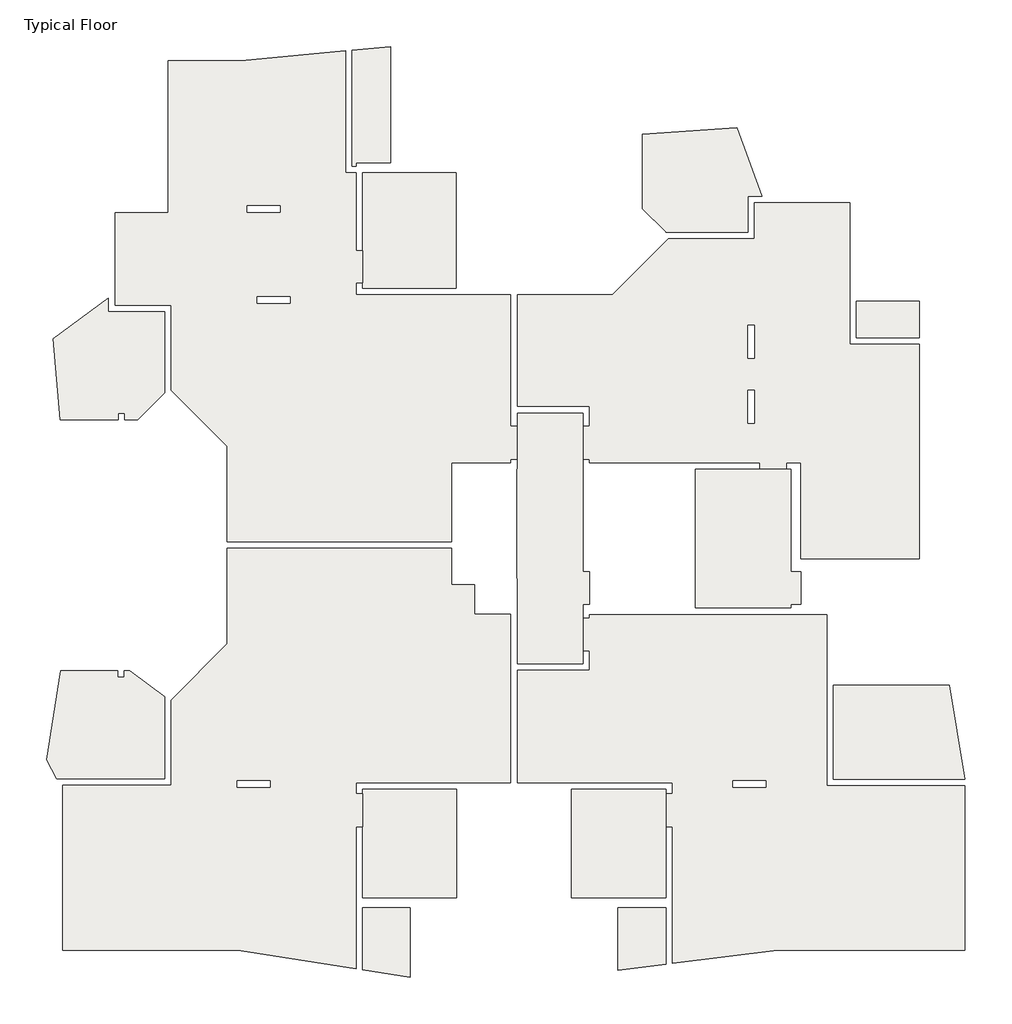
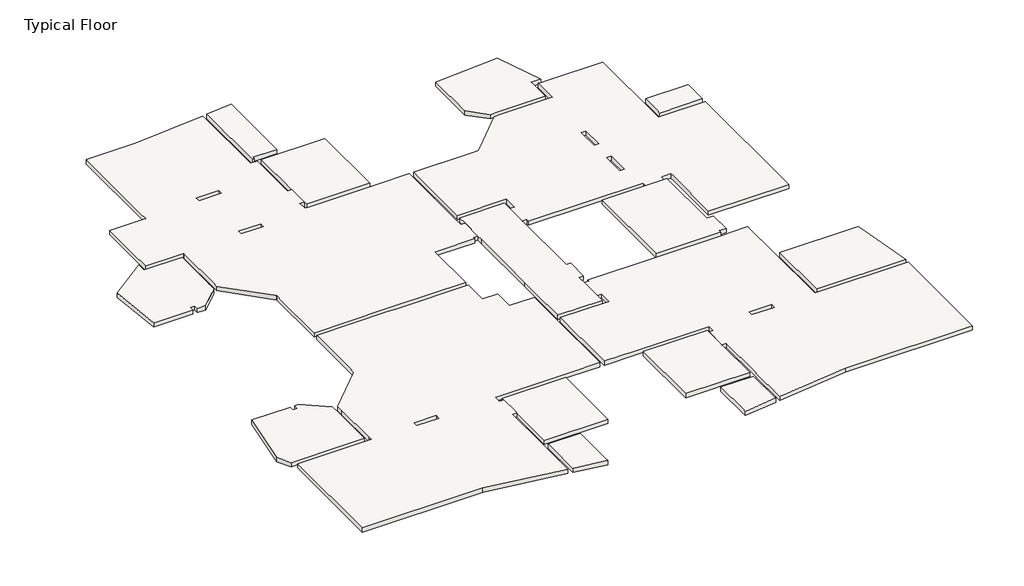
# One storey: 17 slabs.
"""IFC4 building model written with IfcOpenShell, lengths in millimetres."""

from ifc_helpers import new_model, si_unit, origin, place, context, project, spatial, faceted_brep, element, save

model = new_model("IFC4")

# Units and contexts
model_context = context("Model", 3, world=origin())
ifc_project = project(units=[si_unit("LENGTHUNIT", "METRE", prefix="MILLI")], contexts=[model_context])

# Site, building, storey
site = spatial("IfcSite", under=ifc_project)
building = spatial("IfcBuilding", under=site)
storey = spatial("IfcBuildingStorey", under=building, Name="Typical Floor", Elevation=2850.0)

# Slabs
placement = place(None, origin())
element("IfcSlab", 1, ObjectType="20", at=placement, inside=storey, context=model_context, shape_type="Brep", body=[
    faceted_brep([(-15286.5645409, -11765.3513235, 2650.0), (-18561.5127169, -11765.3513235, 2650.0), (-18869.0821124, -11186.8974215, 2650.0), (-18443.4032212, -8499.2666773, 2650.0), (-16708.8112897, -8499.2666773, 2650.0), (-16708.8112897, -8694.3603589, 2650.0), (-16508.8112897, -8694.3603589, 2650.0), (-16508.8112897, -8499.2666773, 2650.0), (-16353.4071605, -8499.2666773, 2650.0), (-15286.5645409, -9274.373211, 2650.0), (-18561.5127169, -11765.3513235, 2850.0), (-18379.347479, -11765.3513235, 2850.0), (-15486.5645409, -11765.3513235, 2850.0), (-15286.5645409, -11765.3513235, 2850.0), (-15286.5645409, -9691.9014804, 2850.0), (-15286.5645409, -9291.9014804, 2850.0), (-15286.5645409, -9274.373211, 2850.0), (-16353.4071605, -8499.2666773, 2850.0), (-16508.8112897, -8499.2666773, 2850.0), (-16508.8112897, -8694.3603589, 2850.0), (-16708.8112897, -8694.3603589, 2850.0), (-16708.8112897, -8499.2666773, 2850.0), (-18443.4032212, -8499.2666773, 2850.0), (-18869.0821124, -11186.8974215, 2850.0)], [[[0, 1, 2, 3, 4, 5, 6, 7, 8, 9]], [[10, 11, 12, 13, 14, 15, 16, 17, 18, 19, 20, 21, 22, 23]], [[1, 0, 13, 12, 11, 10]], [[2, 1, 10, 23]], [[3, 2, 23, 22]], [[4, 3, 22, 21]], [[5, 4, 21, 20]], [[6, 5, 20, 19]], [[7, 6, 19, 18]], [[8, 7, 18, 17]], [[9, 8, 17, 16]], [[0, 9, 16, 15, 14, 13]]]),
])
element("IfcSlab", 2, ObjectType="20", at=placement, inside=storey, context=model_context, shape_type="Brep", body=[
    faceted_brep([(-6440.6856227, -12083.2914692, 2650.0), (-6440.6856227, -15367.9244771, 2650.0), (-9283.9897454, -15367.9244771, 2650.0), (-9283.9897454, -13219.4691321, 2650.0), (-9283.9897454, -12214.5716558, 2650.0), (-9283.9897454, -12083.2914692, 2650.0), (-6440.6856227, -12083.2914692, 2850.0), (-9283.9897454, -12083.2914692, 2850.0), (-9283.9897454, -12214.5716558, 2850.0), (-9283.9897454, -13219.4691321, 2850.0), (-9283.9897454, -15367.9244771, 2850.0), (-6440.6856227, -15367.9244771, 2850.0)], [[[0, 1, 2, 3, 4, 5]], [[6, 7, 8, 9, 10, 11]], [[1, 0, 6, 11]], [[2, 1, 11, 10]], [[5, 4, 3, 2, 10, 9, 8, 7]], [[0, 5, 7, 6]]]),
])
element("IfcSlab", 3, ObjectType="20", at=placement, inside=storey, context=model_context, shape_type="Brep", body=[
    faceted_brep([(-87.6035477, -12083.2914692, 2650.0), (-87.6035477, -12214.5716558, 2650.0), (-87.6035477, -13219.4691321, 2650.0), (-87.6035477, -15367.9244771, 2650.0), (-2954.5902544, -15367.9244771, 2650.0), (-2954.5902544, -12083.2914692, 2650.0), (-87.6035477, -12083.2914692, 2850.0), (-2954.5902544, -12083.2914692, 2850.0), (-2954.5902544, -15367.9244771, 2850.0), (-87.6035477, -15367.9244771, 2850.0), (-87.6035477, -13219.4691321, 2850.0), (-87.6035477, -12214.5716558, 2850.0)], [[[0, 1, 2, 3, 4, 5]], [[6, 7, 8, 9, 10, 11]], [[3, 2, 1, 0, 6, 11, 10, 9]], [[4, 3, 9, 8]], [[5, 4, 8, 7]], [[0, 5, 7, 6]]]),
])
element("IfcSlab", 4, ObjectType="20", at=placement, inside=storey, context=model_context, shape_type="Brep", body=[
    faceted_brep([(-9283.9897454, -15667.9244771, 2650.0), (-7844.4831614, -15667.9244771, 2650.0), (-7844.4831614, -17786.8222268, 2650.0), (-9283.9897454, -17557.8098157, 2650.0), (-9283.9897454, -15667.9244771, 2850.0), (-9283.9897454, -17344.4159012, 2850.0), (-9283.9897454, -17557.8098157, 2850.0), (-7844.4831614, -17786.8222268, 2850.0), (-7844.4831614, -17605.2464942, 2850.0), (-7844.4831614, -15667.9244771, 2850.0)], [[[0, 1, 2, 3]], [[4, 5, 6, 7, 8, 9]], [[1, 0, 4, 9]], [[2, 1, 9, 8, 7]], [[3, 2, 7, 6]], [[0, 3, 6, 5, 4]]]),
])
element("IfcSlab", 5, ObjectType="20", at=placement, inside=storey, context=model_context, shape_type="Brep", body=[
    faceted_brep([(-18379.347479, -16969.7313812, 2650.0), (-18379.347479, -11965.3513235, 2650.0), (-15086.5645409, -11965.3513235, 2650.0), (-15086.5645409, -11765.3513235, 2650.0), (-15089.2187138, -11765.3513235, 2650.0), (-15089.2187138, -9691.9014804, 2650.0), (-15086.5645409, -9691.9014804, 2650.0), (-15086.5645409, -9380.9473819, 2650.0), (-13387.4363964, -7681.8192373, 2650.0), (-13387.4363964, -7281.8192373, 2650.0), (-13387.4363964, -4887.4320305, 2650.0), (-13387.4363964, -4787.4320305, 2650.0), (-6597.6379386, -4787.4320305, 2650.0), (-6597.6379386, -5683.2914692, 2650.0), (-6597.6379386, -5883.2914692, 2650.0), (-5897.6379386, -5883.2914692, 2650.0), (-5897.6379386, -6583.2914692, 2650.0), (-5897.6379386, -6783.2914692, 2650.0), (-4797.6379386, -6783.2914692, 2650.0), (-4797.6379386, -11883.2914692, 2650.0), (-6190.6856227, -11883.2914692, 2650.0), (-9283.9897454, -11883.2914692, 2650.0), (-9483.9897454, -11883.2914692, 2650.0), (-9483.9897454, -12214.5716558, 2650.0), (-9283.9897454, -12214.5716558, 2650.0), (-9283.9897454, -13079.4691321, 2650.0), (-9283.9897454, -13219.4691321, 2650.0), (-9483.9897454, -13219.4691321, 2650.0), (-9483.9897454, -15367.9244771, 2650.0), (-9483.9897454, -15667.9244771, 2650.0), (-9483.9897454, -17344.4159012, 2650.0), (-9483.9897454, -17526.0844321, 2650.0), (-12973.5990213, -16973.3846199, 2650.0), (-12973.5990213, -16969.7313812, 2650.0), (-13373.5990213, -16969.7313812, 2650.0), (-12084.0109343, -12024.8863444, 2650.0), (-12084.0109343, -11824.8863444, 2650.0), (-13084.0109343, -11824.8863444, 2650.0), (-13084.0109343, -12024.8863444, 2650.0), (-18379.347479, -11965.3513235, 2850.0), (-18379.347479, -12165.3513235, 2850.0), (-18379.347479, -16769.7313812, 2850.0), (-18379.347479, -16969.7313812, 2850.0), (-13373.5990213, -16969.7313812, 2850.0), (-12973.5990213, -16969.7313812, 2850.0), (-12973.5990213, -16973.3846199, 2850.0), (-9483.9897454, -17526.0844321, 2850.0), (-9483.9897454, -17344.4159012, 2850.0), (-9483.9897454, -15667.9244771, 2850.0), (-9483.9897454, -15367.9244771, 2850.0), (-9483.9897454, -13219.4691321, 2850.0), (-9283.9897454, -13219.4691321, 2850.0), (-9283.9897454, -13079.4691321, 2850.0), (-9283.9897454, -12214.5716558, 2850.0), (-9483.9897454, -12214.5716558, 2850.0), (-9483.9897454, -11883.2914692, 2850.0), (-9283.9897454, -11883.2914692, 2850.0), (-6190.6856227, -11883.2914692, 2850.0), (-4797.6379386, -11883.2914692, 2850.0), (-4797.6379386, -11683.2914692, 2850.0), (-4797.6379386, -8483.2914692, 2850.0), (-4797.6379386, -8283.2914692, 2850.0), (-4797.6379386, -6783.2914692, 2850.0), (-5897.6379386, -6783.2914692, 2850.0), (-5897.6379386, -6583.2914692, 2850.0), (-5897.6379386, -5883.2914692, 2850.0), (-6597.6379386, -5883.2914692, 2850.0), (-6597.6379386, -5683.2914692, 2850.0), (-6597.6379386, -4787.4320305, 2850.0), (-9795.9008278, -4787.4320305, 2850.0), (-10195.9008278, -4787.4320305, 2850.0), (-13387.4363964, -4787.4320305, 2850.0), (-13387.4363964, -4887.4320305, 2850.0), (-13387.4363964, -7281.8192373, 2850.0), (-13387.4363964, -7681.8192373, 2850.0), (-15086.5645409, -9380.9473819, 2850.0), (-15086.5645409, -9691.9014804, 2850.0), (-15089.2187138, -9691.9014804, 2850.0), (-15089.2187138, -11765.3513235, 2850.0), (-15086.5645409, -11765.3513235, 2850.0), (-15086.5645409, -11965.3513235, 2850.0), (-15486.5645409, -11965.3513235, 2850.0), (-12084.0109343, -11824.8863444, 2850.0), (-12084.0109343, -12024.8863444, 2850.0), (-13084.0109343, -12024.8863444, 2850.0), (-13084.0109343, -11824.8863444, 2850.0)], [[[0, 1, 2, 3, 4, 5, 6, 7, 8, 9, 10, 11, 12, 13, 14, 15, 16, 17, 18, 19, 20, 21, 22, 23, 24, 25, 26, 27, 28, 29, 30, 31, 32, 33, 34], [35, 36, 37, 38]], [[39, 40, 41, 42, 43, 44, 45, 46, 47, 48, 49, 50, 51, 52, 53, 54, 55, 56, 57, 58, 59, 60, 61, 62, 63, 64, 65, 66, 67, 68, 69, 70, 71, 72, 73, 74, 75, 76, 77, 78, 79, 80, 81], [82, 83, 84, 85]], [[1, 0, 42, 41, 40, 39]], [[1, 39, 81, 80, 2]], [[77, 5, 4, 78]], [[74, 8, 7, 75]], [[8, 74, 73, 72, 71, 11, 10, 9]], [[12, 11, 71, 70, 69, 68]], [[12, 68, 67, 66, 14, 13]], [[15, 14, 66, 65]], [[15, 65, 64, 63, 17, 16]], [[18, 17, 63, 62]], [[19, 18, 62, 61, 60, 59, 58]], [[19, 58, 57, 56, 55, 22, 21, 20]], [[23, 22, 55, 54]], [[24, 23, 54, 53]], [[25, 24, 53, 52]], [[26, 25, 52, 51]], [[27, 26, 51, 50]], [[27, 50, 49, 48, 47, 46, 31, 30, 29, 28]], [[32, 31, 46, 45]], [[33, 32, 45, 44]], [[33, 44, 43, 42, 0, 34]], [[6, 76, 75, 7]], [[76, 6, 5, 77]], [[3, 79, 78, 4]], [[79, 3, 2, 80]], [[35, 83, 82, 36]], [[83, 35, 38, 84]], [[84, 38, 37, 85]], [[85, 37, 36, 82]]]),
])
element("IfcSlab", 6, ObjectType="20", at=placement, inside=storey, context=model_context, shape_type="Brep", body=[
    faceted_brep([(8500.876934, -8926.3350173, 2650.0), (8977.0164469, -11773.6548619, 2650.0), (8977.0164469, -11783.2914692, 2650.0), (4985.5431075, -11783.2914692, 2650.0), (4985.5431075, -8926.3350173, 2650.0), (8500.876934, -8926.3350173, 2850.0), (4985.5431075, -8926.3350173, 2850.0), (4985.5431075, -9026.3350173, 2850.0), (4985.5431075, -11583.2914692, 2850.0), (4985.5431075, -11783.2914692, 2850.0), (8977.0164469, -11783.2914692, 2850.0), (8977.0164469, -11773.6548619, 2850.0)], [[[0, 1, 2, 3, 4]], [[5, 6, 7, 8, 9, 10, 11]], [[1, 0, 5, 11]], [[2, 1, 11, 10]], [[3, 2, 10, 9]], [[4, 3, 9, 8, 7, 6]], [[0, 4, 6, 5]]]),
])
element("IfcSlab", 7, ObjectType="20", at=placement, inside=storey, context=model_context, shape_type="Brep", body=[
    faceted_brep([(-4597.6379386, -8483.2914692, 2650.0), (-2403.3824041, -8483.2914692, 2650.0), (-2403.3824041, -8283.2914692, 2650.0), (-2403.3824041, -7883.2914692, 2650.0), (-2603.3824041, -7883.2914692, 2650.0), (-2603.3824041, -6894.6673257, 2650.0), (-2403.3824041, -6894.6673257, 2650.0), (-2403.3824041, -6790.494584, 2650.0), (4785.5431075, -6790.494584, 2650.0), (4785.5431075, -6990.494584, 2650.0), (4785.5431075, -8626.3350173, 2650.0), (4785.5431075, -9026.3350173, 2650.0), (4785.5431075, -11583.2914692, 2650.0), (4785.5431075, -11983.2914692, 2650.0), (4985.5431075, -11983.2914692, 2650.0), (8977.0164469, -11983.2914692, 2650.0), (8977.0164469, -16969.7313812, 2650.0), (3695.6052151, -16969.7313812, 2650.0), (3295.6052151, -16969.7313812, 2650.0), (3289.488953, -16969.7313812, 2650.0), (112.3964523, -17359.8292888, 2650.0), (112.3964523, -17190.4678354, 2650.0), (112.3964523, -15667.9244771, 2650.0), (112.3964523, -15367.9244771, 2650.0), (112.3964523, -13219.4691321, 2650.0), (-87.6035477, -13219.4691321, 2650.0), (-87.6035477, -12214.5716558, 2650.0), (112.3964523, -12214.5716558, 2650.0), (112.3964523, -11883.2914692, 2650.0), (-87.6035477, -11883.2914692, 2650.0), (-3204.5902544, -11883.2914692, 2650.0), (-4597.6379386, -11883.2914692, 2650.0), (2945.6091526, -11824.8863444, 2650.0), (1945.6091526, -11824.8863444, 2650.0), (1945.6091526, -12024.8863444, 2650.0), (2945.6091526, -12024.8863444, 2650.0), (-2403.3824041, -8483.2914692, 2850.0), (-4597.6379386, -8483.2914692, 2850.0), (-4597.6379386, -11683.2914692, 2850.0), (-4597.6379386, -11883.2914692, 2850.0), (-3204.5902544, -11883.2914692, 2850.0), (-87.6035477, -11883.2914692, 2850.0), (112.3964523, -11883.2914692, 2850.0), (112.3964523, -12214.5716558, 2850.0), (-87.6035477, -12214.5716558, 2850.0), (-87.6035477, -13219.4691321, 2850.0), (112.3964523, -13219.4691321, 2850.0), (112.3964523, -15367.9244771, 2850.0), (112.3964523, -15667.9244771, 2850.0), (112.3964523, -17190.4678354, 2850.0), (112.3964523, -17359.8292888, 2850.0), (3289.488953, -16969.7313812, 2850.0), (3295.6052151, -16969.7313812, 2850.0), (3695.6052151, -16969.7313812, 2850.0), (8977.0164469, -16969.7313812, 2850.0), (8977.0164469, -16771.5953491, 2850.0), (8977.0164469, -12165.3513235, 2850.0), (8977.0164469, -11983.2914692, 2850.0), (4985.5431075, -11983.2914692, 2850.0), (4785.5431075, -11983.2914692, 2850.0), (4785.5431075, -11583.2914692, 2850.0), (4785.5431075, -9026.3350173, 2850.0), (4785.5431075, -8626.3350173, 2850.0), (4785.5431075, -6990.494584, 2850.0), (4785.5431075, -6790.494584, 2850.0), (3996.1514357, -6790.494584, 2850.0), (3696.1514357, -6790.494584, 2850.0), (-2403.3824041, -6790.494584, 2850.0), (-2403.3824041, -6894.6673257, 2850.0), (-2603.3824041, -6894.6673257, 2850.0), (-2603.3824041, -7883.2914692, 2850.0), (-2403.3824041, -7883.2914692, 2850.0), (-2403.3824041, -8283.2914692, 2850.0), (1945.6091526, -11824.8863444, 2850.0), (2945.6091526, -11824.8863444, 2850.0), (2945.6091526, -12024.8863444, 2850.0), (1945.6091526, -12024.8863444, 2850.0)], [[[0, 1, 2, 3, 4, 5, 6, 7, 8, 9, 10, 11, 12, 13, 14, 15, 16, 17, 18, 19, 20, 21, 22, 23, 24, 25, 26, 27, 28, 29, 30, 31], [32, 33, 34, 35]], [[36, 37, 38, 39, 40, 41, 42, 43, 44, 45, 46, 47, 48, 49, 50, 51, 52, 53, 54, 55, 56, 57, 58, 59, 60, 61, 62, 63, 64, 65, 66, 67, 68, 69, 70, 71, 72], [73, 74, 75, 76]], [[1, 0, 37, 36]], [[1, 36, 72, 71, 3, 2]], [[4, 3, 71, 70]], [[5, 4, 70, 69]], [[6, 5, 69, 68]], [[7, 6, 68, 67]], [[8, 7, 67, 66, 65, 64]], [[8, 64, 63, 62, 61, 60, 59, 13, 12, 11, 10, 9]], [[13, 59, 58, 57, 15, 14]], [[16, 15, 57, 56, 55, 54]], [[16, 54, 53, 52, 18, 17]], [[19, 18, 52, 51]], [[20, 19, 51, 50]], [[20, 50, 49, 48, 47, 46, 24, 23, 22, 21]], [[25, 24, 46, 45]], [[26, 25, 45, 44]], [[27, 26, 44, 43]], [[28, 27, 43, 42]], [[28, 42, 41, 40, 39, 31, 30, 29]], [[0, 31, 39, 38, 37]], [[33, 32, 74, 73]], [[34, 33, 73, 76]], [[35, 34, 76, 75]], [[32, 35, 75, 74]]]),
])
element("IfcSlab", 8, ObjectType="20", at=placement, inside=storey, context=model_context, shape_type="Brep", body=[
    faceted_brep([(7591.3944084, 2705.1624293, 2650.0), (7591.3944084, 1595.5159248, 2650.0), (5684.9828456, 1595.5159248, 2650.0), (5684.9828456, 2705.1624293, 2650.0), (7591.3944084, 2705.1624293, 2850.0), (5684.9828456, 2705.1624293, 2850.0), (5684.9828456, 1795.5159248, 2850.0), (5684.9828456, 1595.5159248, 2850.0), (7591.3944084, 1595.5159248, 2850.0)], [[[0, 1, 2, 3]], [[4, 5, 6, 7, 8]], [[1, 0, 4, 8]], [[2, 1, 8, 7]], [[3, 2, 7, 6, 5]], [[0, 3, 5, 4]]]),
])
element("IfcSlab", 9, ObjectType="20", at=placement, inside=storey, context=model_context, shape_type="Brep", body=[
    faceted_brep([(-6450.1625371, 3095.9323955, 2650.0), (-9290.6856227, 3095.9323955, 2650.0), (-9290.6856227, 3262.2142639, 2650.0), (-9290.6856227, 4237.8899275, 2650.0), (-9290.6856227, 6597.8899275, 2650.0), (-6450.1625371, 6597.8899275, 2650.0), (-6450.1625371, 3095.9323955, 2850.0), (-6450.1625371, 6597.8899275, 2850.0), (-9290.6856227, 6597.8899275, 2850.0), (-9290.6856227, 4237.8899275, 2850.0), (-9290.6856227, 3262.2142639, 2850.0), (-9290.6856227, 3095.9323955, 2850.0)], [[[0, 1, 2, 3, 4, 5]], [[6, 7, 8, 9, 10, 11]], [[1, 0, 6, 11]], [[4, 3, 2, 1, 11, 10, 9, 8]], [[5, 4, 8, 7]], [[0, 5, 7, 6]]]),
])
element("IfcSlab", 10, ObjectType="20", at=placement, inside=storey, context=model_context, shape_type="Brep", body=[
    faceted_brep([(-9490.6856227, 4237.8899275, 2650.0), (-9290.6856227, 4237.8899275, 2650.0), (-9290.6856227, 3262.2142639, 2650.0), (-9490.6856227, 3262.2142639, 2650.0), (-9490.6856227, 2895.9323955, 2650.0), (-9290.6856227, 2895.9323955, 2650.0), (-6200.1625371, 2895.9323955, 2650.0), (-4797.6379386, 2895.9323955, 2650.0), (-4797.6379386, 2696.2012144, 2650.0), (-4797.6379386, -483.2914692, 2650.0), (-4797.6379386, -1083.2914692, 2650.0), (-4597.6379386, -1083.2914692, 2650.0), (-4597.6379386, -2083.2914692, 2650.0), (-4797.6379386, -2083.2914692, 2650.0), (-4797.6379386, -2183.2914692, 2650.0), (-6397.6379386, -2183.2914692, 2650.0), (-6597.6379386, -2183.2914692, 2650.0), (-6597.6379386, -4587.4320305, 2650.0), (-13387.4363964, -4587.4320305, 2650.0), (-13387.4363964, -4487.4320305, 2650.0), (-13387.4363964, -1688.5879682, 2650.0), (-13388.8740156, -1688.5879682, 2650.0), (-13587.4363964, -1490.0255874, 2650.0), (-15089.2187138, 11.75673, 2650.0), (-15089.2187138, 15.2853334, 2650.0), (-15089.2187138, 316.4585788, 2650.0), (-15089.2187138, 2386.9126556, 2650.0), (-15089.2187138, 2586.9126556, 2650.0), (-15094.2441564, 2586.9126556, 2650.0), (-15489.2187138, 2586.9126556, 2650.0), (-16794.2441564, 2586.9126556, 2650.0), (-16794.2441564, 5384.8420774, 2650.0), (-15386.5645409, 5384.8420774, 2650.0), (-15186.5645409, 5384.8420774, 2650.0), (-15186.5645409, 5784.8420774, 2650.0), (-15186.5645409, 9788.9617999, 2650.0), (-15186.5645409, 9988.9617999, 2650.0), (-13373.5990213, 9988.9617999, 2650.0), (-12973.5990213, 9988.9617999, 2650.0), (-12968.8298625, 9988.9617999, 2650.0), (-9797.9493855, 10292.099937, 2650.0), (-9797.9493855, 10088.7487212, 2650.0), (-9797.9493855, 6598.9542002, 2650.0), (-9490.6856227, 6598.9542002, 2650.0), (-12489.8453542, 2837.5348136, 2650.0), (-12489.8453542, 2637.5348136, 2650.0), (-11489.8453542, 2637.5348136, 2650.0), (-11489.8453542, 2837.5348136, 2650.0), (-12783.7609512, 5596.0878026, 2650.0), (-12783.7609512, 5396.0878026, 2650.0), (-11783.7609512, 5396.0878026, 2650.0), (-11783.7609512, 5596.0878026, 2650.0), (-9290.6856227, 4237.8899275, 2850.0), (-9490.6856227, 4237.8899275, 2850.0), (-9490.6856227, 6598.9542002, 2850.0), (-9797.9493855, 6598.9542002, 2850.0), (-9797.9493855, 6798.9542002, 2850.0), (-9797.9493855, 10088.7487212, 2850.0), (-9797.9493855, 10292.099937, 2850.0), (-12968.8298625, 9988.9617999, 2850.0), (-12973.5990213, 9988.9617999, 2850.0), (-13373.5990213, 9988.9617999, 2850.0), (-15186.5645409, 9988.9617999, 2850.0), (-15186.5645409, 9788.9617999, 2850.0), (-15186.5645409, 5784.8420774, 2850.0), (-15186.5645409, 5384.8420774, 2850.0), (-15386.5645409, 5384.8420774, 2850.0), (-16794.2441564, 5384.8420774, 2850.0), (-16794.2441564, 5184.8420774, 2850.0), (-16794.2441564, 3193.9964468, 2850.0), (-16794.2441564, 2945.4436777, 2850.0), (-16794.2441564, 2786.9126556, 2850.0), (-16794.2441564, 2586.9126556, 2850.0), (-15489.2187138, 2586.9126556, 2850.0), (-15094.2441564, 2586.9126556, 2850.0), (-15089.2187138, 2586.9126556, 2850.0), (-15089.2187138, 2386.9126556, 2850.0), (-15089.2187138, 316.4585788, 2850.0), (-15089.2187138, 11.75673, 2850.0), (-13587.4363964, -1490.0255874, 2850.0), (-13388.8740156, -1688.5879682, 2850.0), (-13387.4363964, -1688.5879682, 2850.0), (-13387.4363964, -2088.5879682, 2850.0), (-13387.4363964, -4487.4320305, 2850.0), (-13387.4363964, -4587.4320305, 2850.0), (-10195.9008278, -4587.4320305, 2850.0), (-9795.9008278, -4587.4320305, 2850.0), (-6597.6379386, -4587.4320305, 2850.0), (-6597.6379386, -2183.2914692, 2850.0), (-6397.6379386, -2183.2914692, 2850.0), (-4797.6379386, -2183.2914692, 2850.0), (-4797.6379386, -2083.2914692, 2850.0), (-4597.6379386, -2083.2914692, 2850.0), (-4597.6379386, -1083.2914692, 2850.0), (-4797.6379386, -1083.2914692, 2850.0), (-4797.6379386, -483.2914692, 2850.0), (-4797.6379386, 2696.2012144, 2850.0), (-4797.6379386, 2895.9323955, 2850.0), (-6200.1625371, 2895.9323955, 2850.0), (-9290.6856227, 2895.9323955, 2850.0), (-9490.6856227, 2895.9323955, 2850.0), (-9490.6856227, 3262.2142639, 2850.0), (-9290.6856227, 3262.2142639, 2850.0), (-12489.8453542, 2637.5348136, 2850.0), (-12489.8453542, 2837.5348136, 2850.0), (-11489.8453542, 2837.5348136, 2850.0), (-11489.8453542, 2637.5348136, 2850.0), (-12783.7609512, 5396.0878026, 2850.0), (-12783.7609512, 5596.0878026, 2850.0), (-11783.7609512, 5596.0878026, 2850.0), (-11783.7609512, 5396.0878026, 2850.0)], [[[0, 1, 2, 3, 4, 5, 6, 7, 8, 9, 10, 11, 12, 13, 14, 15, 16, 17, 18, 19, 20, 21, 22, 23, 24, 25, 26, 27, 28, 29, 30, 31, 32, 33, 34, 35, 36, 37, 38, 39, 40, 41, 42, 43], [44, 45, 46, 47], [48, 49, 50, 51]], [[52, 53, 54, 55, 56, 57, 58, 59, 60, 61, 62, 63, 64, 65, 66, 67, 68, 69, 70, 71, 72, 73, 74, 75, 76, 77, 78, 79, 80, 81, 82, 83, 84, 85, 86, 87, 88, 89, 90, 91, 92, 93, 94, 95, 96, 97, 98, 99, 100, 101, 102], [103, 104, 105, 106], [107, 108, 109, 110]], [[1, 0, 53, 52]], [[2, 1, 52, 102]], [[3, 2, 102, 101]], [[4, 3, 101, 100]], [[4, 100, 99, 98, 97, 7, 6, 5]], [[7, 97, 96, 95, 94, 10, 9, 8]], [[11, 10, 94, 93]], [[12, 11, 93, 92]], [[13, 12, 92, 91]], [[14, 13, 91, 90]], [[14, 90, 89, 88, 16, 15]], [[17, 16, 88, 87]], [[18, 17, 87, 86, 85, 84]], [[18, 84, 83, 82, 81, 20, 19]], [[78, 23, 22, 21, 80, 79]], [[23, 78, 77, 76, 75, 27, 26, 25, 24]], [[28, 27, 75, 74]], [[28, 74, 73, 72, 30, 29]], [[31, 30, 72, 71, 70, 69, 68, 67]], [[31, 67, 66, 65, 33, 32]], [[33, 65, 64, 63, 62, 36, 35, 34]], [[36, 62, 61, 60, 59, 39, 38, 37]], [[40, 39, 59, 58]], [[40, 58, 57, 56, 55, 42, 41]], [[43, 42, 55, 54]], [[0, 43, 54, 53]], [[20, 81, 80, 21]], [[44, 104, 103, 45]], [[104, 44, 47, 105]], [[105, 47, 46, 106]], [[45, 103, 106, 46]], [[48, 108, 107, 49]], [[108, 48, 51, 109]], [[109, 51, 50, 110]], [[49, 107, 110, 50]]]),
])
element("IfcSlab", 11, ObjectType="20", at=placement, inside=storey, context=model_context, shape_type="Brep", body=[
    faceted_brep([(-9597.9493855, 6798.9542002, 2650.0), (-9597.9493855, 10311.2200609, 2650.0), (-8437.0941181, 10422.1985433, 2650.0), (-8437.0941181, 6897.8899275, 2650.0), (-9290.6856227, 6897.8899275, 2650.0), (-9490.6856227, 6897.8899275, 2650.0), (-9490.6856227, 6798.9542002, 2650.0), (-9597.9493855, 10311.2200609, 2850.0), (-9597.9493855, 10088.7487212, 2850.0), (-9597.9493855, 6798.9542002, 2850.0), (-9490.6856227, 6798.9542002, 2850.0), (-9490.6856227, 6897.8899275, 2850.0), (-9290.6856227, 6897.8899275, 2850.0), (-8437.0941181, 6897.8899275, 2850.0), (-8437.0941181, 10222.4041492, 2850.0), (-8437.0941181, 10422.1985433, 2850.0)], [[[0, 1, 2, 3, 4, 5, 6]], [[7, 8, 9, 10, 11, 12, 13, 14, 15]], [[1, 0, 9, 8, 7]], [[2, 1, 7, 15]], [[3, 2, 15, 14, 13]], [[3, 13, 12, 11, 5, 4]], [[6, 5, 11, 10]], [[0, 6, 10, 9]]]),
])
element("IfcSlab", 12, ObjectType="20", at=placement, inside=storey, context=model_context, shape_type="Brep", body=[
    faceted_brep([(-18667.1860705, 1563.4435406, 2650.0), (-16994.2441564, 2797.8683443, 2650.0), (-16994.2441564, 2786.9126556, 2650.0), (-16994.2441564, 2386.9126556, 2650.0), (-16794.2441564, 2386.9126556, 2650.0), (-15489.2187138, 2386.9126556, 2650.0), (-15289.2187138, 2386.9126556, 2650.0), (-15284.2187138, 2386.9126556, 2650.0), (-15284.2187138, 316.4585788, 2650.0), (-15289.2187138, 316.4585788, 2650.0), (-15289.2187138, -73.3367957, 2650.0), (-16107.2350357, -891.3531176, 2650.0), (-16494.0770885, -891.3531176, 2650.0), (-16494.0770885, -691.3531176, 2650.0), (-16694.0770885, -691.3531176, 2650.0), (-16694.0770885, -891.3531176, 2650.0), (-18452.5305511, -891.3531176, 2650.0), (-16994.2441564, 2797.8683443, 2850.0), (-18667.1860705, 1563.4435406, 2850.0), (-18452.5305511, -891.3531176, 2850.0), (-16694.0770885, -891.3531176, 2850.0), (-16694.0770885, -691.3531176, 2850.0), (-16494.0770885, -691.3531176, 2850.0), (-16494.0770885, -891.3531176, 2850.0), (-16107.2350357, -891.3531176, 2850.0), (-15289.2187138, -73.3367957, 2850.0), (-15289.2187138, 316.4585788, 2850.0), (-15284.2187138, 316.4585788, 2850.0), (-15284.2187138, 2386.9126556, 2850.0), (-15489.2187138, 2386.9126556, 2850.0), (-16794.2441564, 2386.9126556, 2850.0), (-16994.2441564, 2386.9126556, 2850.0), (-16994.2441564, 2786.9126556, 2850.0)], [[[0, 1, 2, 3, 4, 5, 6, 7, 8, 9, 10, 11, 12, 13, 14, 15, 16]], [[17, 18, 19, 20, 21, 22, 23, 24, 25, 26, 27, 28, 29, 30, 31, 32]], [[1, 0, 18, 17]], [[1, 17, 32, 31, 3, 2]], [[3, 31, 30, 29, 28, 7, 6, 5, 4]], [[7, 28, 27, 8]], [[24, 11, 10, 25]], [[12, 11, 24, 23]], [[13, 12, 23, 22]], [[14, 13, 22, 21]], [[15, 14, 21, 20]], [[16, 15, 20, 19]], [[0, 16, 19, 18]], [[9, 26, 25, 10]], [[26, 9, 8, 27]]]),
])
element("IfcSlab", 13, ObjectType="20", at=placement, inside=storey, context=model_context, shape_type="Brep", body=[
    faceted_brep([(-799.5327681, 5514.1816932, 2650.0), (-799.5327681, 7759.5088284, 2650.0), (2065.6791891, 7959.8639661, 2650.0), (2826.2618446, 5892.1423364, 2650.0), (2789.104476, 5892.1423364, 2650.0), (2389.104476, 5892.1423364, 2650.0), (2389.104476, 5692.1423364, 2650.0), (2389.104476, 4798.5979252, 2650.0), (-83.949, 4798.5979252, 2650.0), (-799.5327681, 7759.5088284, 2850.0), (-799.5327681, 5514.1816932, 2850.0), (-88.2404871, 4802.8894122, 2850.0), (-83.949, 4798.5979252, 2850.0), (310.22401, 4798.5979252, 2850.0), (2189.104476, 4798.5979252, 2850.0), (2389.104476, 4798.5979252, 2850.0), (2389.104476, 5692.1423364, 2850.0), (2389.104476, 5892.1423364, 2850.0), (2789.104476, 5892.1423364, 2850.0), (2826.2618446, 5892.1423364, 2850.0), (2065.6791891, 7959.8639661, 2850.0)], [[[0, 1, 2, 3, 4, 5, 6, 7, 8]], [[9, 10, 11, 12, 13, 14, 15, 16, 17, 18, 19, 20]], [[1, 0, 10, 9]], [[2, 1, 9, 20]], [[3, 2, 20, 19]], [[3, 19, 18, 17, 5, 4]], [[5, 17, 16, 15, 7, 6]], [[8, 7, 15, 14, 13, 12]], [[0, 8, 12, 11, 10]]]),
])
element("IfcSlab", 14, ObjectType="20", at=placement, inside=storey, context=model_context, shape_type="Brep", body=[
    faceted_brep([(-1699.1198792, 2895.9323955, 2650.0), (-1699.1198792, 2909.1673916, 2650.0), (-9.6893457, 4598.5979252, 2650.0), (310.22401, 4598.5979252, 2650.0), (2189.104476, 4598.5979252, 2650.0), (2589.104476, 4598.5979252, 2650.0), (2589.104476, 4798.5979252, 2650.0), (2589.104476, 5692.1423364, 2650.0), (5484.9828456, 5692.1423364, 2650.0), (5484.9828456, 5494.9383888, 2650.0), (5484.9828456, 1795.5159248, 2650.0), (5484.9828456, 1395.5159248, 2650.0), (5684.9828456, 1395.5159248, 2650.0), (7591.3944084, 1395.5159248, 2650.0), (7591.3944084, -5091.9879156, 2650.0), (3996.1514357, -5091.9879156, 2650.0), (3996.1514357, -2386.1332064, 2650.0), (3996.1514357, -2186.1332064, 2650.0), (3556.6175959, -2186.1332064, 2650.0), (3556.6175959, -2386.1332064, 2650.0), (2756.6175959, -2386.1332064, 2650.0), (2756.6175959, -2186.1332064, 2650.0), (-2403.3824041, -2186.1332064, 2650.0), (-2403.3824041, -2086.1332064, 2650.0), (-2603.3824041, -2086.1332064, 2650.0), (-2603.3824041, -1083.2914692, 2650.0), (-2403.3824041, -1083.2914692, 2650.0), (-2403.3824041, -683.2914692, 2650.0), (-2403.3824041, -483.2914692, 2650.0), (-4597.6379386, -483.2914692, 2650.0), (-4597.6379386, 2895.9323955, 2650.0), (-2099.1198792, 2895.9323955, 2650.0), (2587.619868, 1976.5237192, 2650.0), (2387.619868, 1976.5237192, 2650.0), (2387.619868, 976.5237192, 2650.0), (2587.619868, 976.5237192, 2650.0), (2587.619868, 0.7719728, 2650.0), (2387.619868, 0.7719728, 2650.0), (2387.619868, -999.2280272, 2650.0), (2587.619868, -999.2280272, 2650.0), (-1699.1198792, 2909.1673916, 2850.0), (-1699.1198792, 2895.9323955, 2850.0), (-2099.1198792, 2895.9323955, 2850.0), (-4597.6379386, 2895.9323955, 2850.0), (-4597.6379386, 2696.2012144, 2850.0), (-4597.6379386, -483.2914692, 2850.0), (-2403.3824041, -483.2914692, 2850.0), (-2403.3824041, -683.2914692, 2850.0), (-2403.3824041, -1083.2914692, 2850.0), (-2603.3824041, -1083.2914692, 2850.0), (-2603.3824041, -2086.1332064, 2850.0), (-2403.3824041, -2086.1332064, 2850.0), (-2403.3824041, -2186.1332064, 2850.0), (2756.6175959, -2186.1332064, 2850.0), (2756.6175959, -2386.1332064, 2850.0), (3556.6175959, -2386.1332064, 2850.0), (3556.6175959, -2186.1332064, 2850.0), (3996.1514357, -2186.1332064, 2850.0), (3996.1514357, -2386.1332064, 2850.0), (3996.1514357, -5091.9879156, 2850.0), (7591.3944084, -5091.9879156, 2850.0), (7591.3944084, -4891.9879156, 2850.0), (7591.3944084, -1988.6737606, 2850.0), (7591.3944084, -1588.6737606, 2850.0), (7591.3944084, 1195.5159248, 2850.0), (7591.3944084, 1395.5159248, 2850.0), (5684.9828456, 1395.5159248, 2850.0), (5484.9828456, 1395.5159248, 2850.0), (5484.9828456, 1795.5159248, 2850.0), (5484.9828456, 5494.9383888, 2850.0), (5484.9828456, 5692.1423364, 2850.0), (3112.9302979, 5692.1423364, 2850.0), (2899.8290642, 5692.1423364, 2850.0), (2789.104476, 5692.1423364, 2850.0), (2589.104476, 5692.1423364, 2850.0), (2589.104476, 4798.5979252, 2850.0), (2589.104476, 4598.5979252, 2850.0), (2189.104476, 4598.5979252, 2850.0), (310.22401, 4598.5979252, 2850.0), (-9.6893457, 4598.5979252, 2850.0), (-1512.3548709, 3095.9324, 2850.0), (2387.619868, 0.7719728, 2850.0), (2587.619868, 0.7719728, 2850.0), (2587.619868, -999.2280272, 2850.0), (2387.619868, -999.2280272, 2850.0), (2387.619868, 1976.5237192, 2850.0), (2587.619868, 1976.5237192, 2850.0), (2587.619868, 976.5237192, 2850.0), (2387.619868, 976.5237192, 2850.0)], [[[0, 1, 2, 3, 4, 5, 6, 7, 8, 9, 10, 11, 12, 13, 14, 15, 16, 17, 18, 19, 20, 21, 22, 23, 24, 25, 26, 27, 28, 29, 30, 31], [32, 33, 34, 35], [36, 37, 38, 39]], [[40, 41, 42, 43, 44, 45, 46, 47, 48, 49, 50, 51, 52, 53, 54, 55, 56, 57, 58, 59, 60, 61, 62, 63, 64, 65, 66, 67, 68, 69, 70, 71, 72, 73, 74, 75, 76, 77, 78, 79, 80], [81, 82, 83, 84], [85, 86, 87, 88]], [[41, 0, 31, 30, 43, 42]], [[1, 0, 41, 40]], [[2, 1, 40, 80, 79]], [[2, 79, 78, 77, 76, 5, 4, 3]], [[5, 76, 75, 74, 7, 6]], [[8, 7, 74, 73, 72, 71, 70]], [[8, 70, 69, 68, 67, 11, 10, 9]], [[11, 67, 66, 65, 13, 12]], [[14, 13, 65, 64, 63, 62, 61, 60]], [[15, 14, 60, 59]], [[15, 59, 58, 57, 17, 16]], [[18, 17, 57, 56]], [[19, 18, 56, 55]], [[20, 19, 55, 54]], [[21, 20, 54, 53]], [[22, 21, 53, 52]], [[23, 22, 52, 51]], [[24, 23, 51, 50]], [[25, 24, 50, 49]], [[26, 25, 49, 48]], [[26, 48, 47, 46, 28, 27]], [[29, 28, 46, 45]], [[30, 29, 45, 44, 43]], [[33, 32, 86, 85]], [[34, 33, 85, 88]], [[35, 34, 88, 87]], [[32, 35, 87, 86]], [[37, 36, 82, 81]], [[38, 37, 81, 84]], [[39, 38, 84, 83]], [[36, 39, 83, 82]]]),
])
element("IfcSlab", 15, ObjectType="20", at=placement, inside=storey, context=model_context, shape_type="Brep", body=[
    faceted_brep([(3696.1514357, -2386.1332064, 2650.0), (3696.1514357, -5486.1332064, 2650.0), (3996.1514357, -5486.1332064, 2650.0), (3996.1514357, -6470.494584, 2650.0), (3696.1514357, -6470.494584, 2650.0), (3696.1514357, -6590.494584, 2650.0), (796.6175959, -6590.494584, 2650.0), (796.6175959, -2386.1332064, 2650.0), (2756.6175959, -2386.1332064, 2650.0), (3556.6175959, -2386.1332064, 2650.0), (3696.1514357, -5486.1332064, 2850.0), (3696.1514357, -2386.1332064, 2850.0), (3556.6175959, -2386.1332064, 2850.0), (2756.6175959, -2386.1332064, 2850.0), (796.6175959, -2386.1332064, 2850.0), (796.6175959, -6590.494584, 2850.0), (3696.1514357, -6590.494584, 2850.0), (3696.1514357, -6470.494584, 2850.0), (3996.1514357, -6470.494584, 2850.0), (3996.1514357, -5486.1332064, 2850.0)], [[[0, 1, 2, 3, 4, 5, 6, 7, 8, 9]], [[10, 11, 12, 13, 14, 15, 16, 17, 18, 19]], [[1, 0, 11, 10]], [[2, 1, 10, 19]], [[3, 2, 19, 18]], [[4, 3, 18, 17]], [[5, 4, 17, 16]], [[6, 5, 16, 15]], [[7, 6, 15, 14]], [[7, 14, 13, 12, 11, 0, 9, 8]]]),
])
element("IfcSlab", 16, ObjectType="20", at=placement, inside=storey, context=model_context, shape_type="Brep", body=[
    faceted_brep([(-2403.3824041, -6474.6673257, 2650.0), (-2603.3824041, -6474.6673257, 2650.0), (-2603.3824041, -6894.6673257, 2650.0), (-2603.3824041, -7883.2914692, 2650.0), (-2603.3824041, -8283.2914692, 2650.0), (-4597.6379386, -8283.2914692, 2650.0), (-4597.6379386, -5683.2914692, 2650.0), (-4602.6379386, -5683.2914692, 2650.0), (-4602.6379386, -2383.2914692, 2650.0), (-4597.6379386, -2383.2914692, 2650.0), (-4597.6379386, -2083.2914692, 2650.0), (-4597.6379386, -1083.2914692, 2650.0), (-4597.6379386, -683.2914692, 2650.0), (-2603.3824041, -683.2914692, 2650.0), (-2603.3824041, -1083.2914692, 2650.0), (-2603.3824041, -2086.1332064, 2650.0), (-2603.3824041, -5486.1332064, 2650.0), (-2403.3824041, -5486.1332064, 2650.0), (-2603.3824041, -6474.6673257, 2850.0), (-2403.3824041, -6474.6673257, 2850.0), (-2403.3824041, -5486.1332064, 2850.0), (-2603.3824041, -5486.1332064, 2850.0), (-2603.3824041, -2086.1332064, 2850.0), (-2603.3824041, -1083.2914692, 2850.0), (-2603.3824041, -683.2914692, 2850.0), (-4597.6379386, -683.2914692, 2850.0), (-4597.6379386, -1083.2914692, 2850.0), (-4597.6379386, -2083.2914692, 2850.0), (-4597.6379386, -2383.2914692, 2850.0), (-4602.6379386, -2383.2914692, 2850.0), (-4602.6379386, -5683.2914692, 2850.0), (-4597.6379386, -5683.2914692, 2850.0), (-4597.6379386, -6583.2914692, 2850.0), (-4597.6379386, -8283.2914692, 2850.0), (-2603.3824041, -8283.2914692, 2850.0), (-2603.3824041, -7883.2914692, 2850.0), (-2603.3824041, -6894.6673257, 2850.0)], [[[0, 1, 2, 3, 4, 5, 6, 7, 8, 9, 10, 11, 12, 13, 14, 15, 16, 17]], [[18, 19, 20, 21, 22, 23, 24, 25, 26, 27, 28, 29, 30, 31, 32, 33, 34, 35, 36]], [[13, 24, 23, 22, 21, 16, 15, 14]], [[4, 34, 33, 5]], [[29, 8, 7, 30]], [[24, 13, 12, 25]], [[19, 0, 17, 20]], [[1, 0, 19, 18]], [[2, 1, 18, 36]], [[4, 3, 35, 34]], [[3, 2, 36, 35]], [[9, 28, 27, 26, 25, 12, 11, 10]], [[28, 9, 8, 29]], [[16, 21, 20, 17]], [[5, 33, 32, 31, 6]], [[6, 31, 30, 7]]]),
])
element("IfcSlab", 17, ObjectType="20", at=placement, inside=storey, context=model_context, shape_type="Brep", body=[
    faceted_brep([(-87.6035477, -15667.9244771, 2650.0), (-87.6035477, -17384.386201, 2650.0), (-1546.410046, -17563.5051163, 2650.0), (-1546.410046, -15667.9244771, 2650.0), (-87.6035477, -17384.386201, 2850.0), (-87.6035477, -17190.4678354, 2850.0), (-87.6035477, -15667.9244771, 2850.0), (-1546.410046, -15667.9244771, 2850.0), (-1546.410046, -17401.7807651, 2850.0), (-1546.410046, -17563.5051163, 2850.0)], [[[0, 1, 2, 3]], [[4, 5, 6, 7, 8, 9]], [[1, 0, 6, 5, 4]], [[2, 1, 4, 9]], [[3, 2, 9, 8, 7]], [[0, 3, 7, 6]]]),
])

save(model, "model.ifc")

# Revit data of these elements
# Type "20"
#   Function = 0
#   Layers, outside or top first: 20 cm "Concrete" (function 1)
# Element 1 (IfcSlab, "20")
#   Mark = "S1"
#   SOFiSTiK_AMG_Comments = ""
#   Height Offset From Level = 0 cm
#   built-in parameter 1001954 = 1
#   SOFiSTiK_AMG_Scheduled = yes
#   SOFiSTiK_AMG_Adjusted = no
#   Phase Created = New Construction
#   Materials on its faces: "Concrete"
# Element 2 (IfcSlab, "20")
#   Mark = "S2"
#   SOFiSTiK_AMG_Comments = ""
#   Height Offset From Level = 0 cm
#   built-in parameter 1001954 = 1
#   SOFiSTiK_AMG_Scheduled = yes
#   SOFiSTiK_AMG_Adjusted = yes
#   Phase Created = New Construction
#   Materials on its faces: "Concrete"
# Element 3 (IfcSlab, "20")
#   Mark = "S3"
#   SOFiSTiK_AMG_Comments = ""
#   Height Offset From Level = 0 cm
#   built-in parameter 1001954 = 1
#   SOFiSTiK_AMG_Scheduled = yes
#   SOFiSTiK_AMG_Adjusted = yes
#   Phase Created = New Construction
#   Materials on its faces: "Concrete"
# Element 4 (IfcSlab, "20")
#   Mark = "S4"
#   SOFiSTiK_AMG_Comments = ""
#   built-in parameter 1001955 = 1.5708 (stored number, unit not read)
#   Height Offset From Level = 0 cm
#   built-in parameter 1001954 = 1
#   SOFiSTiK_AMG_Scheduled = yes
#   SOFiSTiK_AMG_Adjusted = yes
#   Phase Created = New Construction
#   Materials on its faces: "Concrete"
# Element 5 (IfcSlab, "20")
#   Mark = "S5"
#   SOFiSTiK_AMG_Comments = ""
#   built-in parameter 1001955 = -1.5708 (stored number, unit not read)
#   Height Offset From Level = 0 cm
#   built-in parameter 1001954 = 1
#   SOFiSTiK_AMG_Scheduled = yes
#   SOFiSTiK_AMG_Adjusted = yes
#   Phase Created = New Construction
#   Materials on its faces: "Concrete"
# Element 6 (IfcSlab, "20")
#   Mark = "S6"
#   SOFiSTiK_AMG_Comments = ""
#   Height Offset From Level = 0 cm
#   built-in parameter 1001954 = 1
#   SOFiSTiK_AMG_Scheduled = yes
#   SOFiSTiK_AMG_Adjusted = yes
#   Phase Created = New Construction
#   Materials on its faces: "Concrete"
# Element 7 (IfcSlab, "20")
#   Mark = "S7"
#   SOFiSTiK_AMG_Comments = ""
#   built-in parameter 1001955 = 1.5708 (stored number, unit not read)
#   Height Offset From Level = 0 cm
#   built-in parameter 1001954 = 1
#   SOFiSTiK_AMG_Scheduled = yes
#   SOFiSTiK_AMG_Adjusted = no
#   Phase Created = New Construction
#   Materials on its faces: "Concrete"
# Element 8 (IfcSlab, "20")
#   Mark = "S8"
#   SOFiSTiK_AMG_Comments = ""
#   Height Offset From Level = 0 cm
#   built-in parameter 1001954 = 1
#   SOFiSTiK_AMG_Scheduled = yes
#   SOFiSTiK_AMG_Adjusted = yes
#   Phase Created = New Construction
#   Materials on its faces: "Concrete"
# Element 9 (IfcSlab, "20")
#   Mark = "S9"
#   SOFiSTiK_AMG_Comments = ""
#   Height Offset From Level = 0 cm
#   built-in parameter 1001954 = 1
#   SOFiSTiK_AMG_Scheduled = yes
#   SOFiSTiK_AMG_Adjusted = yes
#   Phase Created = New Construction
#   Materials on its faces: "Concrete"
# Element 10 (IfcSlab, "20")
#   Mark = "S10"
#   SOFiSTiK_AMG_Comments = ""
#   built-in parameter 1001955 = 3.14159 (stored number, unit not read)
#   Height Offset From Level = 0 cm
#   built-in parameter 1001954 = 1
#   SOFiSTiK_AMG_Scheduled = yes
#   SOFiSTiK_AMG_Adjusted = no
#   Phase Created = New Construction
#   Materials on its faces: "Concrete"
# Element 11 (IfcSlab, "20")
#   Mark = "S11"
#   SOFiSTiK_AMG_Comments = ""
#   built-in parameter 1001955 = 3.14159 (stored number, unit not read)
#   Height Offset From Level = 0 cm
#   built-in parameter 1001954 = 1
#   SOFiSTiK_AMG_Scheduled = yes
#   SOFiSTiK_AMG_Adjusted = yes
#   Phase Created = New Construction
#   Materials on its faces: "Concrete"
# Element 12 (IfcSlab, "20")
#   Mark = "S12"
#   SOFiSTiK_AMG_Comments = ""
#   built-in parameter 1001955 = -2.5059 (stored number, unit not read)
#   Height Offset From Level = 0 cm
#   built-in parameter 1001954 = 1
#   SOFiSTiK_AMG_Scheduled = yes
#   SOFiSTiK_AMG_Adjusted = no
#   Phase Created = New Construction
#   Materials on its faces: "Concrete"
# Element 13 (IfcSlab, "20")
#   Mark = "S13"
#   SOFiSTiK_AMG_Comments = ""
#   built-in parameter 1001955 = 2.35619 (stored number, unit not read)
#   Height Offset From Level = 0 cm
#   built-in parameter 1001954 = 1
#   SOFiSTiK_AMG_Scheduled = yes
#   SOFiSTiK_AMG_Adjusted = yes
#   Phase Created = New Construction
#   Materials on its faces: "Concrete"
# Element 14 (IfcSlab, "20")
#   Mark = "S14"
#   SOFiSTiK_AMG_Comments = ""
#   built-in parameter 1001955 = 1.5708 (stored number, unit not read)
#   Height Offset From Level = 0 cm
#   built-in parameter 1001954 = 1
#   SOFiSTiK_AMG_Scheduled = yes
#   SOFiSTiK_AMG_Adjusted = yes
#   Phase Created = New Construction
#   Materials on its faces: "Concrete"
# Element 15 (IfcSlab, "20")
#   Mark = "S15"
#   SOFiSTiK_AMG_Comments = ""
#   Height Offset From Level = 0 cm
#   built-in parameter 1001954 = 1
#   SOFiSTiK_AMG_Scheduled = yes
#   SOFiSTiK_AMG_Adjusted = yes
#   Phase Created = New Construction
#   Materials on its faces: "Concrete"
# Element 16 (IfcSlab, "20")
#   Mark = "S16"
#   SOFiSTiK_AMG_Comments = ""
#   Height Offset From Level = 0 cm
#   built-in parameter 1001954 = 1
#   SOFiSTiK_AMG_Scheduled = yes
#   SOFiSTiK_AMG_Adjusted = yes
#   Phase Created = New Construction
#   Materials on its faces: "Concrete"
# Element 17 (IfcSlab, "20")
#   Mark = "S17"
#   SOFiSTiK_AMG_Comments = ""
#   Height Offset From Level = 0 cm
#   built-in parameter 1001954 = 1
#   SOFiSTiK_AMG_Scheduled = yes
#   SOFiSTiK_AMG_Adjusted = yes
#   Phase Created = New Construction
#   Materials on its faces: "Concrete"
# Materials
#   "Concrete": class "Concrete", colour RGB 192 192 192, transparency 0, Keynote = "01000", Description = "Cast-in-place concrete", Cost = 0
